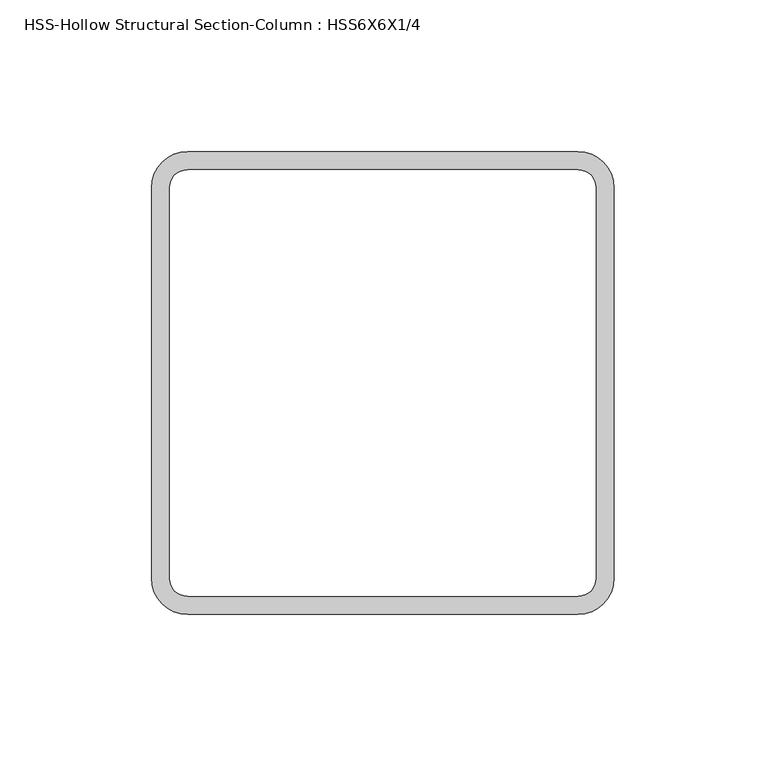
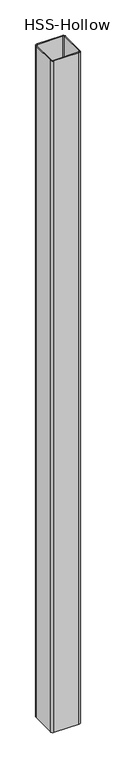
"""IFC4 building model written with IfcOpenShell, lengths in millimetres: column geometry, HSS-Hollow Structural Section-Column : HSS6X6X1/4."""

import ifcopenshell
import ifcopenshell.guid

model = None  # the IFC model being written
_history = None  # IfcOwnerHistory: only IFC2X3 demands one
_inside = {}  # id of a spatial element -> (the spatial element, [elements in it])
_under = {}  # id of a project, library or spatial element -> (it, [spatial elements below it])
_declared = {}  # id of a project -> (the project, [libraries it declares])
_typed = {}  # id of a type object -> (the type object, [elements of that type])
_made_of = {}  # id of a material, layer set ... -> (it, [elements and type objects made of it])


def new_model(schema):
    """Start an empty IFC model of exactly this schema.

    Asked for "IFC4X3", IfcOpenShell would pick the latest addendum, in which some entities
    have other attributes; the version numbers below select the first issue.
    IFC2X3 requires an IfcOwnerHistory on every rooted entity: one is made here for all.
    """
    global model, _history
    if schema == "IFC4X3":
        model = ifcopenshell.file(schema_version=(4, 3, 0, 0))
    else:
        model = ifcopenshell.file(schema=schema)
    _inside.clear()
    _under.clear()
    _declared.clear()
    _typed.clear()
    _made_of.clear()
    _history = None
    if model.schema == "IFC2X3":
        org = make("IfcOrganization", Name="unknown")
        user = make(
            "IfcPersonAndOrganization",
            ThePerson=make("IfcPerson", FamilyName="unknown"),
            TheOrganization=org,
        )
        app = make(
            "IfcApplication",
            ApplicationDeveloper=org,
            Version="unknown",
            ApplicationFullName="unknown",
            ApplicationIdentifier="unknown",
        )
        _history = make(
            "IfcOwnerHistory",
            OwningUser=user,
            OwningApplication=app,
            ChangeAction="ADDED",
            CreationDate=0,
        )
    return model


def make(cls, **values):
    """One entity of the class cls with the attributes given. An attribute that is None is left unset."""
    return model.create_entity(
        cls, **{name: value for name, value in values.items() if value is not None}
    )


def rooted(cls, **values):
    """An entity with a GlobalId (a new one), such as an element, a storey or a relation."""
    return make(cls, GlobalId=ifcopenshell.guid.new(), OwnerHistory=_history, **values)


def si_unit(unit_type, name, prefix=None):
    """IfcSIUnit, for example si_unit("LENGTHUNIT", "METRE", prefix="MILLI")."""
    return make("IfcSIUnit", UnitType=unit_type, Prefix=prefix, Name=name)


def assignment(units):
    """IfcUnitAssignment: the units of a project."""
    return None if units is None else make("IfcUnitAssignment", Units=units)


def point(xyz):
    """IfcCartesianPoint."""
    return None if xyz is None else make("IfcCartesianPoint", Coordinates=xyz)


def direction(xyz):
    """IfcDirection."""
    return None if xyz is None else make("IfcDirection", DirectionRatios=xyz)


def frame(location, z_axis=None, x_axis=None):
    """IfcAxis2Placement3D, a coordinate frame: its origin and axes. An axis left out is left unset."""
    return make(
        "IfcAxis2Placement3D",
        Location=point(location),
        Axis=direction(z_axis),
        RefDirection=direction(x_axis),
    )


def frame_2d(location, x_axis=None):
    """IfcAxis2Placement2D, a coordinate frame in the plane: its origin and x axis."""
    return make(
        "IfcAxis2Placement2D", Location=point(location), RefDirection=direction(x_axis)
    )


def origin():
    """The frame at (0, 0, 0) with its axes left unset."""
    return frame((0.0, 0.0, 0.0))


def origin_with_axes():
    """The frame at (0, 0, 0) with the z axis (0, 0, 1) and the x axis (1, 0, 0) written out."""
    return frame((0.0, 0.0, 0.0), z_axis=(0.0, 0.0, 1.0), x_axis=(1.0, 0.0, 0.0))


def place(relative_to, where):
    """IfcLocalPlacement: puts the frame where relative to a parent placement (None: the world)."""
    return make(
        "IfcLocalPlacement", PlacementRelTo=relative_to, RelativePlacement=where
    )


def context(
    kind, dimensions, precision=None, world=None, true_north=None, identifier=None
):
    """IfcGeometricRepresentationContext, for example the 3D "Model" context."""
    return make(
        "IfcGeometricRepresentationContext",
        ContextIdentifier=identifier,
        ContextType=kind,
        CoordinateSpaceDimension=dimensions,
        Precision=precision,
        WorldCoordinateSystem=world,
        TrueNorth=true_north,
    )


def project(units=None, contexts=None):
    """IfcProject with its units and contexts."""
    return rooted(
        "IfcProject",
        Name="project",
        RepresentationContexts=contexts,
        UnitsInContext=assignment(units),
    )


def spatial(cls, under=None, at=None, **own):
    """A site, building, storey or space (cls), placed at a placement, below another one or the project."""
    s = rooted(cls, ObjectPlacement=at, **own)
    if under is not None:
        _under.setdefault(under.id(), (under, []))[1].append(s)
    return s


def polyline(points):
    """IfcPolyline through the points."""
    return make("IfcPolyline", Points=[point(p) for p in points])


def circle_curve(where, radius):
    """IfcCircle in the frame where."""
    return make("IfcCircle", Position=where, Radius=radius)


def trimmed(basis, trim1, trim2, sense, master):
    """IfcTrimmedCurve: the piece of a basis curve between two trims."""
    return make(
        "IfcTrimmedCurve",
        BasisCurve=basis,
        Trim1=trim1,
        Trim2=trim2,
        SenseAgreement=sense,
        MasterRepresentation=master,
    )


def segment(curve, same_sense, transition):
    """IfcCompositeCurveSegment."""
    return make(
        "IfcCompositeCurveSegment",
        Transition=transition,
        SameSense=same_sense,
        ParentCurve=curve,
    )


def composite_curve(segments, self_intersect=None):
    """IfcCompositeCurve: segments joined end to end."""
    return make("IfcCompositeCurve", Segments=segments, SelfIntersect=self_intersect)


def outline(outer, holes=None, kind="AREA"):
    """IfcArbitraryClosedProfileDef: a profile drawn as a closed curve; with holes, ...WithVoids."""
    if holes is None:
        return make("IfcArbitraryClosedProfileDef", ProfileType=kind, OuterCurve=outer)
    return make(
        "IfcArbitraryProfileDefWithVoids",
        ProfileType=kind,
        OuterCurve=outer,
        InnerCurves=holes,
    )


def extrude(swept, where, along, depth):
    """IfcExtrudedAreaSolid: the profile swept, set in the frame where, extruded along a direction by depth."""
    return make(
        "IfcExtrudedAreaSolid",
        SweptArea=swept,
        Position=where,
        ExtrudedDirection=direction(along),
        Depth=depth,
    )


def shape(context_of_items, identifier, shape_type, items):
    """IfcShapeRepresentation: the items that make up one representation, for example the "Body"."""
    return make(
        "IfcShapeRepresentation",
        ContextOfItems=context_of_items,
        RepresentationIdentifier=identifier,
        RepresentationType=shape_type,
        Items=items,
    )


def source(mapping_origin, context_of_items, identifier, shape_type, items):
    """IfcRepresentationMap: a shape defined once, which mapped items show again and again."""
    return make(
        "IfcRepresentationMap",
        MappingOrigin=mapping_origin,
        MappedRepresentation=shape(context_of_items, identifier, shape_type, items),
    )


def transform(
    local_origin,
    x_axis=None,
    y_axis=None,
    z_axis=None,
    scale=None,
    scale2=None,
    scale3=None,
    uniform=True,
):
    """IfcCartesianTransformationOperator3D, or its non-uniform kind. x_axis, y_axis, z_axis: its Axis1, 2, 3."""
    if uniform:
        return make(
            "IfcCartesianTransformationOperator3D",
            Axis1=direction(x_axis),
            Axis2=direction(y_axis),
            LocalOrigin=point(local_origin),
            Scale=scale,
            Axis3=direction(z_axis),
        )
    return make(
        "IfcCartesianTransformationOperator3DnonUniform",
        Axis1=direction(x_axis),
        Axis2=direction(y_axis),
        LocalOrigin=point(local_origin),
        Scale=scale,
        Axis3=direction(z_axis),
        Scale2=scale2,
        Scale3=scale3,
    )


def mapped(mapping_source, mapping_target):
    """IfcMappedItem: shows the shape of a source again, moved by a transform."""
    return make(
        "IfcMappedItem", MappingSource=mapping_source, MappingTarget=mapping_target
    )


def made_of(thing, what):
    """Note that an element or type object is made of a material, layer set ...; save() writes the relation."""
    if what is not None:
        _made_of.setdefault(what.id(), (what, []))[1].append(thing)
    return thing


def element(
    cls,
    number,
    at=None,
    inside=None,
    cuts=None,
    type_object=None,
    material=None,
    context=None,
    identifier="Body",
    shape_type=None,
    held_by="IfcProductDefinitionShape",
    body=None,
    shapes=None,
    **own,
):
    """One element of the class cls, such as IfcWall. Its Tag is "e" and its number.

    at: its placement. inside: the storey or other place that contains it. cuts: it is an
    opening in that element (IfcRelVoidsElement). A single representation is given by context,
    identifier, shape_type and body (its items); several are given by shapes. held_by: the class
    of the entity that holds the representations. save() writes the other relations.
    """
    e = rooted(cls, Tag="e%d" % number, ObjectPlacement=at, **own)
    if body is not None:
        shapes = [shape(context, identifier, shape_type, body)]
    if shapes is not None:
        e.Representation = make(held_by, Representations=shapes)
    if inside is not None:
        _inside.setdefault(inside.id(), (inside, []))[1].append(e)
    if cuts is not None:
        rooted(
            "IfcRelVoidsElement", RelatingBuildingElement=cuts, RelatedOpeningElement=e
        )
    if type_object is not None:
        _typed.setdefault(type_object.id(), (type_object, []))[1].append(e)
    return made_of(e, material)


def aggregate(whole, parts):
    """IfcRelAggregates: a whole, such as a stair, and the parts it consists of."""
    return rooted("IfcRelAggregates", RelatingObject=whole, RelatedObjects=parts)


def save(model, path):
    """Write the relations noted so far, then the file.

    IfcRelAggregates (storeys below a building ...), IfcRelContainedInSpatialStructure (elements
    in a storey), IfcRelDefinesByType, IfcRelAssociatesMaterial and IfcRelDeclares: one each for
    every whole, place, type object, material and project.
    """
    for whole, parts in _under.values():
        aggregate(whole, parts)
    for where, things in _inside.values():
        rooted(
            "IfcRelContainedInSpatialStructure",
            RelatedElements=things,
            RelatingStructure=where,
        )
    for kind, things in _typed.values():
        rooted("IfcRelDefinesByType", RelatedObjects=things, RelatingType=kind)
    for what, things in _made_of.values():
        rooted("IfcRelAssociatesMaterial", RelatedObjects=things, RelatingMaterial=what)
    for by, libraries in _declared.values():
        rooted("IfcRelDeclares", RelatingContext=by, RelatedDefinitions=libraries)
    model.write(path)


def hss_hollow_structural_section_column_hss6x6x1_4_de73236b(model_context):
    return source(origin(), model_context, "Body", "SweptSolid", [
        extrude(outline(composite_curve([segment(trimmed(circle_curve(frame_2d((64.3636, 64.3636)), 11.8364), [point((64.3636, 76.2))], [point((76.2, 64.3636))], False, "CARTESIAN"), True, "CONTINUOUS"), segment(polyline([(76.2, 64.3636), (76.2, -64.3636)]), True, "CONTINUOUS"), segment(trimmed(circle_curve(frame_2d((64.3636, -64.3636)), 11.8364), [point((76.2, -64.3636))], [point((64.3636, -76.2))], False, "CARTESIAN"), True, "CONTINUOUS"), segment(polyline([(64.3636, -76.2), (-64.3636, -76.2)]), True, "CONTINUOUS"), segment(trimmed(circle_curve(frame_2d((-64.3636, -64.3636)), 11.8364), [point((-64.3636, -76.2))], [point((-76.2, -64.3636))], False, "CARTESIAN"), True, "CONTINUOUS"), segment(polyline([(-76.2, -64.3636), (-76.2, 64.3636)]), True, "CONTINUOUS"), segment(trimmed(circle_curve(frame_2d((-64.3636, 64.3636)), 11.8364), [point((-76.2, 64.3636))], [point((-64.3636, 76.2))], False, "CARTESIAN"), True, "CONTINUOUS"), segment(polyline([(-64.3636, 76.2), (64.3636, 76.2)]), True, "CONTINUOUS")], self_intersect=False), holes=[composite_curve([segment(polyline([(64.3636, 70.2818), (-64.3636, 70.2818)]), True, "CONTINUOUS"), segment(trimmed(circle_curve(frame_2d((-64.3636, 64.3636)), 5.9182), [point((-64.3636, 70.2818))], [point((-70.2818, 64.3636))], True, "CARTESIAN"), True, "CONTINUOUS"), segment(polyline([(-70.2818, 64.3636), (-70.2818, -64.3636)]), True, "CONTINUOUS"), segment(trimmed(circle_curve(frame_2d((-64.3636, -64.3636)), 5.9182), [point((-70.2818, -64.3636))], [point((-64.3636, -70.2818))], True, "CARTESIAN"), True, "CONTINUOUS"), segment(polyline([(-64.3636, -70.2818), (64.3636, -70.2818)]), True, "CONTINUOUS"), segment(trimmed(circle_curve(frame_2d((64.3636, -64.3636)), 5.9182), [point((64.3636, -70.2818))], [point((70.2818, -64.3636))], True, "CARTESIAN"), True, "CONTINUOUS"), segment(polyline([(70.2818, -64.3636), (70.2818, 64.3636)]), True, "CONTINUOUS"), segment(trimmed(circle_curve(frame_2d((64.3636, 64.3636)), 5.9182), [point((70.2818, 64.3636))], [point((64.3636, 70.2818))], True, "CARTESIAN"), True, "CONTINUOUS")], self_intersect=False)]), origin_with_axes(), (0.0, 0.0, 1.0), 3657.6),
    ])


if __name__ == "__main__":
    model = new_model("IFC4")
    model_context = context("Model", 3, world=origin())
    ifc_project = project(units=[si_unit("LENGTHUNIT", "METRE", prefix="MILLI")], contexts=[model_context])
    site = spatial("IfcSite", under=ifc_project)
    building = spatial("IfcBuilding", under=site)
    placement = place(None, origin())
    hss_hollow_structural_section_column_hss6x6x1_4_shape = hss_hollow_structural_section_column_hss6x6x1_4_de73236b(model_context)
    element("IfcColumn", 1, ObjectType="HSS-Hollow Structural Section-Column : HSS6X6X1/4", at=placement, inside=building, context=model_context, shape_type="MappedRepresentation", body=[
        mapped(hss_hollow_structural_section_column_hss6x6x1_4_shape, transform((0.0, 0.0, 0.0), x_axis=(1.0, 0.0, 0.0), y_axis=(0.0, 1.0, 0.0), z_axis=(0.0, 0.0, 1.0))),
    ])
    save(model, "model.ifc")

# Revit data of these elements
# Type "HSS-Hollow Structural Section-Column : HSS6X6X1/4"
#   Assembly Code = "B10"
#   Shape = "Square"
#   W = 19
#   Ht = 0' - 6"
#   b = 0' - 6"
#   kr = 0' - 0.466"
#   t = 0' - 0.233"
#   A = 0.0363889 SF
#   Structural Material [instance default] = Steel ASTM A500, Grade B, Rectangular and Square
# Element 1 (IfcColumn, "HSS-Hollow Structural Section-Column : HSS6X6X1/4")
#   Structural Material = Steel
#   Materials on its faces: "Steel"
# Materials
#   "Steel ASTM A500, Grade B, Rectangular and Square": class "Metal", colour RGB 199 199 199, transparency 0, Description = "Carbon steel", Cost = 0
#   "Steel": class "Metal", colour RGB 118 118 114, transparency 0, Description = "Steel, mill finish", Cost = 0
